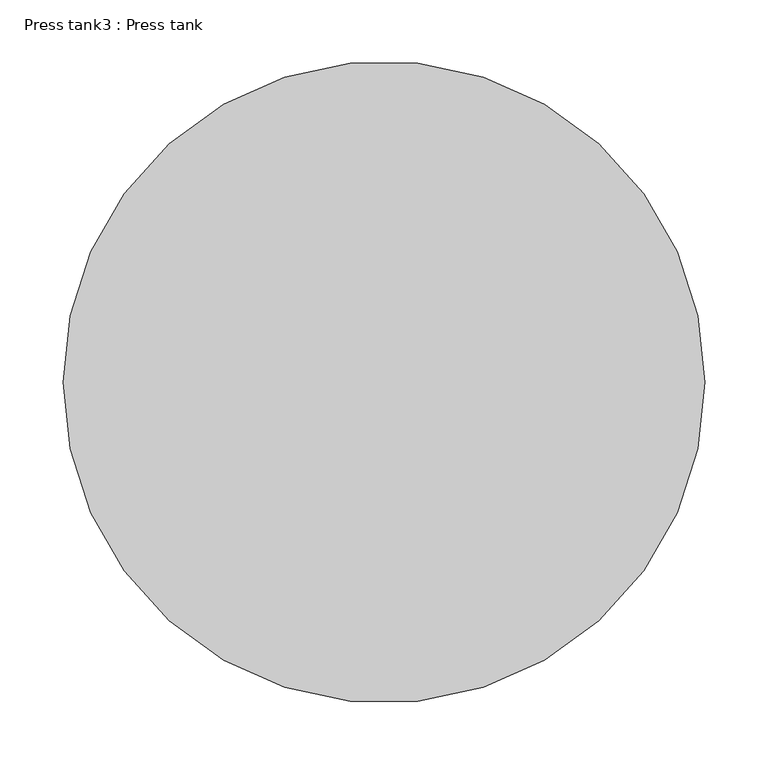
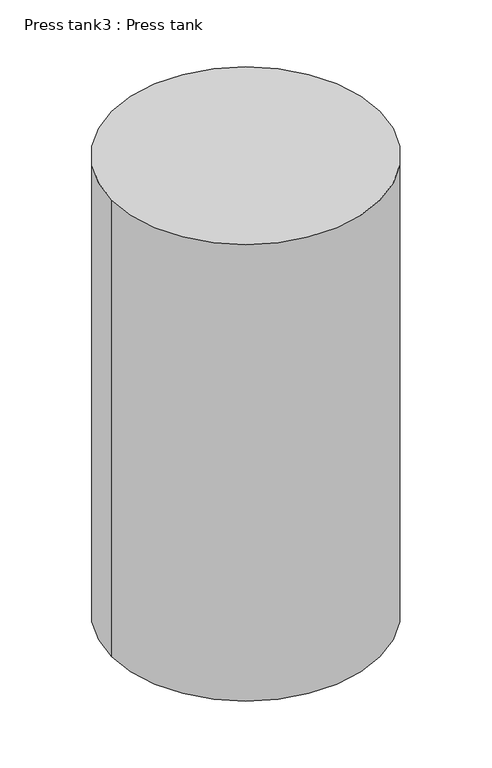
"""IFC4 building model written with IfcOpenShell, lengths in millimetres: proxy geometry, Press tank3 : Press tank."""

from ifc_helpers import new_model, si_unit, point, frame, frame_2d, origin, place, context, project, spatial, circle_curve, trimmed, segment, composite_curve, outline, extrude, source, transform, mapped, element, save


def press_tank3_press_tank_732dd890(model_context):
    return source(origin(), model_context, "Body", "SweptSolid", [
        extrude(outline(composite_curve([segment(trimmed(circle_curve(frame_2d((26385.9004782, 10738.3240491)), 254.0), [point((26131.9004782, 10738.3240491))], [point((26639.9004782, 10738.3240491))], False, "CARTESIAN"), True, "CONTINUOUS"), segment(trimmed(circle_curve(frame_2d((26385.9004782, 10738.3240491)), 254.0), [point((26639.9004782, 10738.3240491))], [point((26131.9004782, 10738.3240491))], False, "CARTESIAN"), True, "CONTINUOUS")], self_intersect=False)), frame((0.0, 0.0, 2832.1), z_axis=(0.0, 0.0, 1.0), x_axis=(1.0, 0.0, 0.0)), (0.0, 0.0, 1.0), 914.4),
    ])


if __name__ == "__main__":
    model = new_model("IFC4")
    model_context = context("Model", 3, world=origin())
    ifc_project = project(units=[si_unit("LENGTHUNIT", "METRE", prefix="MILLI")], contexts=[model_context])
    site = spatial("IfcSite", under=ifc_project)
    building = spatial("IfcBuilding", under=site)
    placement = place(None, origin())
    press_tank3_press_tank_shape = press_tank3_press_tank_732dd890(model_context)
    element("IfcBuildingElementProxy", 1, Name="Press tank3 : Press tank", ObjectType="Press tank3 : Press tank", at=placement, inside=building, context=model_context, shape_type="MappedRepresentation", body=[
        mapped(press_tank3_press_tank_shape, transform((0.0, 0.0, 0.0), x_axis=(1.0, 0.0, 0.0), y_axis=(0.0, 1.0, 0.0), z_axis=(0.0, 0.0, 1.0))),
    ])
    save(model, "model.ifc")
